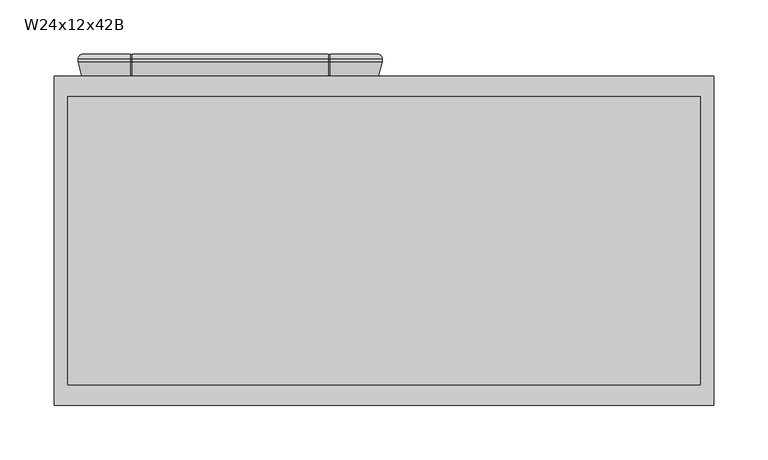
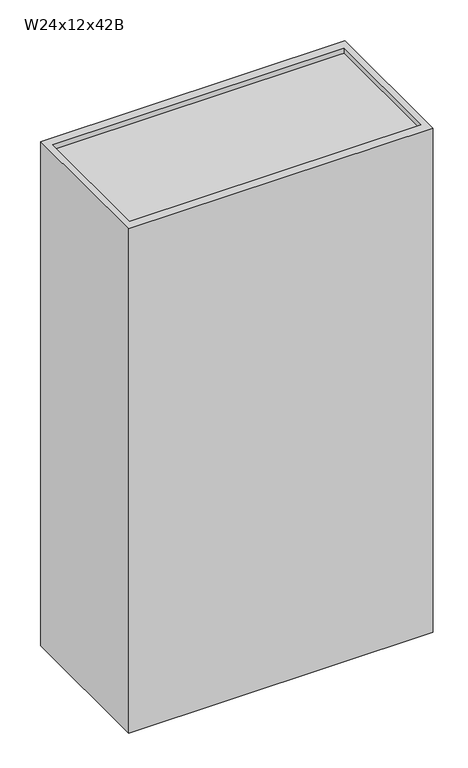
"""IFC4 building model written with IfcOpenShell, lengths in millimetres: furniture geometry, Cabinet-Wall-Merillat-Double_Door-Marlin : W24x12x42B."""

from ifc_helpers import new_model, si_unit, frame, origin, place, context, project, spatial, polyline, circle_curve, ellipse_curve, outline, extrude, faceted_brep, source, transform, mapped, element, save
from ifc_brep_helpers import plane_surface, cylinder_surface, advanced_brep


def w24x12x42b_d67e2903(model_context):
    return source(origin(), model_context, "Body", "SolidModel", [
        advanced_brep(
        [(-24.0971608, 382.5621, 2108.2), (-21.0006683, 387.0325, 2105.1035075), (-21.0006683, 387.0325, 1095.2964925), (-24.0971608, 382.5621, 1092.2), (-24.0971608, 379.7935, 1092.2), (-24.0971608, 379.7935, 2108.2), (-20.5919608, 366.7125, 1095.7052), (-20.5919608, 366.7125, 2104.6948), (24.104002, 366.7125, 2059.9988372), (24.104002, 366.7125, 1140.4011628), (24.4741337, 367.50625, 1140.7712945), (26.5552927, 371.96931, 1142.8524535), (26.5552927, 371.96931, 2057.5475465), (24.4741337, 367.50625, 2059.6287055), (25.1555233, 374.2094093, 1141.452684), (25.1555233, 374.2094093, 2058.947316), (10.8278392, 374.4595, 1127.125), (10.8278392, 374.4595, 2073.275), (10.8278392, 379.2855, 1127.125), (10.8278392, 379.2855, 2073.275), (25.1555233, 379.5355907, 1141.452684), (25.1555233, 379.5355907, 2058.947316), (26.5552927, 381.77569, 1142.8524535), (26.5552927, 381.77569, 2057.5475465), (24.4741337, 386.23875, 1140.7712945), (24.1068694, 387.0263508, 1140.4040302), (24.104002, 387.0325, 2059.9988372), (24.4741337, 386.23875, 2059.6287055), (24.1068694, 387.0325, 1095.2964925), (24.1068694, 382.5621, 1092.2), (253.7938467, 387.0325, 1095.2964925), (256.8903392, 382.5621, 1092.2), (208.7261206, 382.5621, 1092.2), (208.7261206, 387.0325, 1095.2964925), (25.6943694, 382.5621, 1092.2), (25.6943694, 387.0325, 1095.2964925), (207.1386206, 387.0325, 1095.2964925), (207.1386206, 382.5621, 1092.2), (24.1068694, 379.7935, 1092.2), (256.8903392, 379.7935, 1092.2), (208.7261206, 379.7935, 1092.2), (25.6943694, 379.7935, 1092.2), (207.1386206, 379.7935, 1092.2), (24.1068694, 366.7125, 1095.7052), (253.3851392, 366.7125, 1095.7052), (208.7261206, 366.7125, 1095.7052), (25.6943694, 366.7125, 1095.7052), (207.1386206, 366.7125, 1095.7052), (206.2378857, 371.96931, 1142.8524535), (25.6943694, 367.50625, 1140.7712945), (25.6943694, 366.7125, 1140.4011628), (207.1386206, 366.7125, 1140.4011628), (207.1386206, 367.50625, 1140.7712945), (208.3190448, 367.50625, 1140.7712945), (207.6376552, 374.2094093, 1141.452684), (221.9653392, 374.4595, 1127.125), (221.9653392, 379.2855, 1127.125), (207.6376552, 379.5355907, 1141.452684), (206.2378857, 381.77569, 1142.8524535), (208.3190448, 386.23875, 1140.7712945), (207.1386206, 386.23875, 1140.7712945), (207.1386206, 387.0325, 1140.4011628), (25.6943694, 387.0325, 1140.4011628), (25.6943694, 386.23875, 1140.7712945), (253.7938467, 387.0325, 2105.1035075), (256.8903392, 382.5621, 2108.2), (256.8903392, 379.7935, 2108.2), (253.3851392, 366.7125, 2104.6948), (208.6891765, 366.7125, 1140.4011628), (208.6891765, 366.7125, 2059.9988372), (208.3190448, 367.50625, 2059.6287055), (206.2378857, 371.96931, 2057.5475465), (207.6376552, 374.2094093, 2058.947316), (221.9653392, 374.4595, 2073.275), (221.9653392, 379.2855, 2073.275), (207.6376552, 379.5355907, 2058.947316), (206.2378857, 381.77569, 2057.5475465), (208.3190448, 386.23875, 2059.6287055), (208.6891765, 387.0325, 2059.9988372), (208.6891765, 387.0325, 1140.4011628), (208.7261206, 387.0325, 2105.1035075), (208.7261206, 382.5621, 2108.2), (24.1068694, 382.5621, 2108.2), (24.1068694, 387.0325, 2105.1035075), (207.1386206, 382.5621, 2108.2), (207.1386206, 387.0325, 2105.1035075), (25.6943694, 387.0325, 2105.1035075), (25.6943694, 382.5621, 2108.2), (208.7261206, 379.7935, 2108.2), (24.1068694, 379.7935, 2108.2), (207.1386206, 379.7935, 2108.2), (25.6943694, 379.7935, 2108.2), (208.7261206, 366.7125, 2104.6948), (24.1068694, 366.7125, 2104.6948), (207.1386206, 366.7125, 2104.6948), (25.6943694, 366.7125, 2104.6948), (207.1386206, 366.7125, 2059.9988372), (25.6943694, 366.7125, 2059.9988372), (207.1386206, 367.50625, 2059.6287055), (25.6943694, 367.50625, 2059.6287055), (25.6943694, 386.23875, 2059.6287055), (25.6943694, 387.0325, 2059.9988372), (207.1386206, 387.0325, 2059.9988372), (207.1386206, 386.23875, 2059.6287055), (207.1386206, 367.50625, 2104.0857412), (207.1386206, 379.8980037, 2107.40625), (207.1386206, 382.5621, 2107.40625), (207.1386206, 386.23875, 2104.9526052), (208.7261206, 386.23875, 2059.6287055), (208.7261206, 386.23875, 2104.9526052), (208.7261206, 382.5621, 2107.40625), (208.7261206, 379.8980037, 2107.40625), (208.7261206, 367.50625, 2104.0857412), (208.7261206, 367.50625, 2059.6287055), (24.1068694, 367.50625, 2059.6287055), (24.1068694, 367.50625, 2104.0857412), (24.1068694, 379.8980037, 2107.40625), (24.1068694, 382.5621, 2107.40625), (24.1068694, 386.23875, 2104.9526052), (24.1068694, 386.23875, 2059.6287055), (25.6943694, 386.23875, 2104.9526052), (25.6943694, 382.5621, 2107.40625), (25.6943694, 379.8980037, 2107.40625), (25.6943694, 367.50625, 2104.0857412), (24.1068694, 386.23875, 1140.7712945), (24.1068694, 386.23875, 1095.4473948), (24.1068694, 382.5621, 1092.99375), (24.1068694, 379.8980037, 1092.99375), (24.1068694, 367.50625, 1096.3142588), (24.1068694, 367.50625, 1140.7712945), (25.6943694, 367.50625, 1096.3142588), (25.6943694, 379.8980037, 1092.99375), (25.6943694, 382.5621, 1092.99375), (25.6943694, 386.23875, 1095.4473948), (207.1386206, 386.23875, 1095.4473948), (207.1386206, 382.5621, 1092.99375), (207.1386206, 379.8980037, 1092.99375), (207.1386206, 367.50625, 1096.3142588), (208.7261206, 386.23875, 1140.7712945), (208.7261206, 367.50625, 1140.7712945), (208.7261206, 367.50625, 1096.3142588), (208.7261206, 379.8980037, 1092.99375), (208.7261206, 382.5621, 1092.99375), (208.7261206, 386.23875, 1095.4473948)],
        [
            (0, 1, ellipse_curve(frame((-19.3219608, 382.5621, 2103.4248), z_axis=(-0.7071067811865475, 0.0, -0.7071067811865475), x_axis=(-0.7071067811865474, 0.0, 0.7071067811865476)), 6.7531526, 4.7752)),
            (1, 2),
            (2, 3, ellipse_curve(frame((-19.3219608, 382.5621, 1096.9752), z_axis=(-0.7071067811865475, 0.0, 0.7071067811865475), x_axis=(0.7071067811865474, 0.0, 0.7071067811865476)), 6.7531526, 4.7752)),
            (3, 0),
            (3, 4),
            (4, 5),
            (5, 0),
            (4, 6),
            (6, 7),
            (7, 5),
            (8, 9),
            (9, 10),
            (10, 11),
            (11, 12),
            (12, 13),
            (13, 8),
            (11, 14, ellipse_curve(frame((25.1280392, 372.6348492, 1141.4252), z_axis=(-0.7071067811865475, 0.0, 0.7071067811865475), x_axis=(0.7071067811865474, 0.0, 0.7071067811865476)), 2.2271035, 1.5748)),
            (14, 15),
            (15, 12, ellipse_curve(frame((25.1280392, 372.6348492, 2058.9748), z_axis=(-0.7071067811865475, 0.0, -0.7071067811865475), x_axis=(-0.7071067811865474, 0.0, 0.7071067811865476)), 2.2271035, 1.5748)),
            (14, 16),
            (16, 17),
            (17, 15),
            (16, 18),
            (18, 19),
            (19, 17),
            (18, 20),
            (20, 21),
            (21, 19),
            (20, 22, ellipse_curve(frame((25.1280392, 381.1101508, 1141.4252), z_axis=(-0.7071067811865475, 0.0, 0.7071067811865475), x_axis=(0.7071067811865474, 0.0, 0.7071067811865476)), 2.2271035, 1.5748)),
            (22, 23),
            (23, 21, ellipse_curve(frame((25.1280392, 381.1101508, 2058.9748), z_axis=(-0.7071067811865475, 0.0, -0.7071067811865475), x_axis=(-0.7071067811865474, 0.0, 0.7071067811865476)), 2.2271035, 1.5748)),
            (22, 24),
            (24, 25),
            (25, 26),
            (26, 27),
            (27, 23),
            (2, 28),
            (28, 29, circle_curve(frame((24.1068694, 382.5621, 1096.9752), z_axis=(-1.0, 0.0, 0.0), x_axis=(0.0, -1.0, 0.0)), 4.7752)),
            (29, 3),
            (30, 31, ellipse_curve(frame((252.1151392, 382.5621, 1096.9752), z_axis=(-0.7071067811865475, 0.0, -0.7071067811865475), x_axis=(-0.7071067811865476, 0.0, 0.7071067811865474)), 6.7531526, 4.7752)),
            (31, 32),
            (32, 33, circle_curve(frame((208.7261206, 382.5621, 1096.9752), z_axis=(1.0, 0.0, 0.0), x_axis=(0.0, -1.0, 0.0)), 4.7752)),
            (33, 30),
            (34, 35, circle_curve(frame((25.6943694, 382.5621, 1096.9752), z_axis=(1.0, 0.0, 0.0), x_axis=(0.0, -1.0, 0.0)), 4.7752)),
            (35, 36),
            (36, 37, circle_curve(frame((207.1386206, 382.5621, 1096.9752), z_axis=(-1.0, 0.0, 0.0), x_axis=(0.0, -1.0, 0.0)), 4.7752)),
            (37, 34),
            (29, 38),
            (38, 4),
            (31, 39),
            (39, 40),
            (40, 32),
            (41, 34),
            (37, 42),
            (42, 41),
            (38, 43),
            (43, 6),
            (39, 44),
            (44, 45),
            (45, 40),
            (46, 41),
            (42, 47),
            (47, 46),
            (48, 11),
            (10, 49),
            (49, 50),
            (50, 51),
            (51, 52),
            (52, 53),
            (53, 48),
            (48, 54, ellipse_curve(frame((207.6651392, 372.6348492, 1141.4252), z_axis=(-0.7071067811865475, 0.0, -0.7071067811865475), x_axis=(-0.7071067811865476, 0.0, 0.7071067811865474)), 2.2271035, 1.5748)),
            (54, 14),
            (54, 55),
            (55, 16),
            (55, 56),
            (56, 18),
            (56, 57),
            (57, 20),
            (57, 58, ellipse_curve(frame((207.6651392, 381.1101508, 1141.4252), z_axis=(-0.7071067811865475, 0.0, -0.7071067811865475), x_axis=(-0.7071067811865476, 0.0, 0.7071067811865474)), 2.2271035, 1.5748)),
            (58, 22),
            (58, 59),
            (59, 60),
            (60, 61),
            (61, 62),
            (62, 63),
            (63, 24),
            (30, 64),
            (64, 65, ellipse_curve(frame((252.1151392, 382.5621, 2103.4248), z_axis=(0.7071067811865475, 0.0, -0.7071067811865475), x_axis=(-0.7071067811865474, 0.0, -0.7071067811865476)), 6.7531526, 4.7752)),
            (65, 31),
            (65, 66),
            (66, 39),
            (66, 67),
            (67, 44),
            (68, 69),
            (69, 70),
            (70, 71),
            (71, 48),
            (53, 68),
            (71, 72, ellipse_curve(frame((207.6651392, 372.6348492, 2058.9748), z_axis=(0.7071067811865475, 0.0, -0.7071067811865475), x_axis=(-0.7071067811865474, 0.0, -0.7071067811865476)), 2.2271035, 1.5748)),
            (72, 54),
            (72, 73),
            (73, 55),
            (73, 74),
            (74, 56),
            (74, 75),
            (75, 57),
            (75, 76, ellipse_curve(frame((207.6651392, 381.1101508, 2058.9748), z_axis=(0.7071067811865475, 0.0, -0.7071067811865475), x_axis=(-0.7071067811865474, 0.0, -0.7071067811865476)), 2.2271035, 1.5748)),
            (76, 58),
            (76, 77),
            (77, 78),
            (78, 79),
            (79, 59),
            (64, 80),
            (80, 81, circle_curve(frame((208.7261206, 382.5621, 2103.4248), z_axis=(1.0, 0.0, 0.0), x_axis=(0.0, -1.0, 0.0)), 4.7752)),
            (81, 65),
            (0, 82),
            (82, 83, circle_curve(frame((24.1068694, 382.5621, 2103.4248), z_axis=(-1.0, 0.0, 0.0), x_axis=(0.0, -1.0, 0.0)), 4.7752)),
            (83, 1),
            (84, 85, circle_curve(frame((207.1386206, 382.5621, 2103.4248), z_axis=(-1.0, 0.0, 0.0), x_axis=(0.0, -1.0, 0.0)), 4.7752)),
            (85, 86),
            (86, 87, circle_curve(frame((25.6943694, 382.5621, 2103.4248), z_axis=(1.0, 0.0, 0.0), x_axis=(0.0, -1.0, 0.0)), 4.7752)),
            (87, 84),
            (81, 88),
            (88, 66),
            (5, 89),
            (89, 82),
            (90, 84),
            (87, 91),
            (91, 90),
            (88, 92),
            (92, 67),
            (7, 93),
            (93, 89),
            (94, 90),
            (91, 95),
            (95, 94),
            (43, 9),
            (8, 93),
            (92, 69),
            (68, 45),
            (96, 94),
            (95, 97),
            (97, 96),
            (50, 46),
            (47, 51),
            (12, 71),
            (70, 98),
            (98, 96),
            (97, 99),
            (99, 13),
            (15, 72),
            (17, 73),
            (19, 74),
            (21, 75),
            (23, 76),
            (27, 100),
            (100, 101),
            (101, 102),
            (102, 103),
            (103, 77),
            (83, 26),
            (25, 28),
            (33, 79),
            (78, 80),
            (85, 102),
            (101, 86),
            (35, 62),
            (61, 36),
            (98, 104),
            (104, 105),
            (105, 106),
            (106, 107, circle_curve(frame((207.1386206, 382.5621, 2103.4248), z_axis=(-1.0, 0.0, 0.0), x_axis=(0.0, 0.0, 1.0)), 3.98145)),
            (107, 103),
            (78, 108),
            (108, 109),
            (109, 110, circle_curve(frame((208.7261206, 382.5621, 2103.4248), z_axis=(1.0, 0.0, 0.0), x_axis=(0.0, 0.0, 1.0)), 3.98145)),
            (110, 111),
            (111, 112),
            (112, 113),
            (113, 69),
            (77, 108),
            (107, 109),
            (106, 110),
            (105, 111),
            (104, 112),
            (70, 113),
            (8, 114),
            (114, 115),
            (115, 116),
            (116, 117),
            (117, 118, circle_curve(frame((24.1068694, 382.5621, 2103.4248), z_axis=(-1.0, 0.0, 0.0), x_axis=(0.0, 0.0, 1.0)), 3.98145)),
            (118, 119),
            (119, 26),
            (100, 120),
            (120, 121, circle_curve(frame((25.6943694, 382.5621, 2103.4248), z_axis=(1.0, 0.0, 0.0), x_axis=(0.0, 0.0, 1.0)), 3.98145)),
            (121, 122),
            (122, 123),
            (123, 99),
            (119, 27),
            (118, 120),
            (117, 121),
            (116, 122),
            (115, 123),
            (114, 13),
            (25, 124),
            (124, 125),
            (125, 126, circle_curve(frame((24.1068694, 382.5621, 1096.9752), z_axis=(-1.0, 0.0, 0.0), x_axis=(0.0, 0.0, 1.0)), 3.98145)),
            (126, 127),
            (127, 128),
            (128, 129),
            (129, 9),
            (49, 130),
            (130, 131),
            (131, 132),
            (132, 133, circle_curve(frame((25.6943694, 382.5621, 1096.9752), z_axis=(1.0, 0.0, 0.0), x_axis=(0.0, 0.0, 1.0)), 3.98145)),
            (133, 63),
            (129, 10),
            (128, 130),
            (127, 131),
            (126, 132),
            (125, 133),
            (124, 24),
            (60, 134),
            (134, 135, circle_curve(frame((207.1386206, 382.5621, 1096.9752), z_axis=(-1.0, 0.0, 0.0), x_axis=(0.0, 0.0, 1.0)), 3.98145)),
            (135, 136),
            (136, 137),
            (137, 52),
            (138, 79),
            (68, 139),
            (139, 140),
            (140, 141),
            (141, 142),
            (142, 143, circle_curve(frame((208.7261206, 382.5621, 1096.9752), z_axis=(1.0, 0.0, 0.0), x_axis=(0.0, 0.0, 1.0)), 3.98145)),
            (143, 138),
            (138, 59),
            (53, 139),
            (137, 140),
            (136, 141),
            (135, 142),
            (134, 143),
        ],
        [
            cylinder_surface(frame((-19.3219608, 382.5621, 2108.2), z_axis=(0.0, 0.0, 1.0), x_axis=(0.0, -1.0, 0.0)), 4.7752),
            plane_surface(frame((-24.0971608, 382.5621, 2108.2), z_axis=(-1.0, 0.0, 0.0), x_axis=(0.0, 0.0, -1.0))),
            plane_surface(frame((-24.0971608, 379.7935, 2108.2), z_axis=(-0.9659229350723619, -0.25882983502910506, 0.0), x_axis=(0.0, 0.0, -1.0))),
            plane_surface(frame((24.104002, 366.7125, 2059.9988372), z_axis=(0.9063077870366099, -0.4226182617407856, 0.0), x_axis=(0.0, 0.0, -1.0))),
            cylinder_surface(frame((25.1280392, 372.6348492, 2108.2), z_axis=(0.0, 0.0, 1.0000000000000002), x_axis=(0.01745240643729364, 0.9998476951563912, 0.0)), 1.5748),
            plane_surface(frame((25.1555233, 374.2094093, 2058.947316), z_axis=(0.017452406437322144, 0.9998476951563906, 0.0), x_axis=(0.0, 0.0, -1.0))),
            plane_surface(frame((10.8278392, 374.4595, 2073.275), z_axis=(1.0, 0.0, 0.0), x_axis=(0.0, 0.0, -1.0))),
            plane_surface(frame((10.8278392, 379.2855, 2073.275), z_axis=(0.01745240643727848, -0.9998476951563914, 0.0), x_axis=(0.0, 0.0, -1.0))),
            cylinder_surface(frame((25.1280392, 381.1101508, 2108.2), z_axis=(0.0, 0.0, 1.0000000000000002), x_axis=(0.9063077870367326, 0.42261826174052236, 0.0)), 1.5748),
            plane_surface(frame((26.5552927, 381.77569, 2057.5475465), z_axis=(0.9063077870366333, 0.4226182617407352, 0.0), x_axis=(0.0, 0.0, -1.0))),
            cylinder_surface(frame((-24.0971608, 382.5621, 1096.9752), z_axis=(-1.0, 0.0, 0.0), x_axis=(0.0, -1.0, 0.0)), 4.7752),
            plane_surface(frame((-24.0971608, 382.5621, 1092.2), z_axis=(0.0, 0.0, -1.0), x_axis=(1.0, 0.0, 0.0))),
            plane_surface(frame((-24.0971608, 379.7935, 1092.2), z_axis=(0.0, -0.2588298350291095, -0.9659229350723607), x_axis=(1.0, 0.0, 0.0))),
            plane_surface(frame((24.104002, 366.7125, 1140.4011628), z_axis=(0.0, -0.42261826174078143, 0.9063077870366119), x_axis=(1.0, 0.0, 0.0))),
            cylinder_surface(frame((-24.0971608, 372.6348492, 1141.4252), z_axis=(-1.0000000000000002, 0.0, 0.0), x_axis=(0.0, 0.9998476951563913, 0.017452406437289025)), 1.5748),
            plane_surface(frame((25.1555233, 374.2094093, 1141.452684), z_axis=(0.0, 0.9998476951563907, 0.01745240643731753), x_axis=(1.0, 0.0, 0.0))),
            plane_surface(frame((10.8278392, 374.4595, 1127.125), z_axis=(0.0, 0.0, 1.0), x_axis=(1.0, 0.0, 0.0))),
            plane_surface(frame((10.8278392, 379.2855, 1127.125), z_axis=(0.0, -0.9998476951563913, 0.017452406437283095), x_axis=(1.0, 0.0, 0.0))),
            cylinder_surface(frame((-24.0971608, 381.1101508, 1141.4252), z_axis=(-1.0000000000000002, 0.0, 0.0), x_axis=(0.0, 0.4226182617405265, 0.9063077870367306)), 1.5748),
            plane_surface(frame((26.5552927, 381.77569, 1142.8524535), z_axis=(0.0, 0.4226182617407394, 0.9063077870366314), x_axis=(1.0, 0.0, 0.0))),
            cylinder_surface(frame((252.1151392, 382.5621, 1092.2), z_axis=(0.0, 0.0, -1.0), x_axis=(0.0, -1.0, 0.0)), 4.7752),
            plane_surface(frame((256.8903392, 382.5621, 1092.2), z_axis=(1.0, 0.0, 0.0), x_axis=(0.0, 0.0, 1.0))),
            plane_surface(frame((256.8903392, 379.7935, 1092.2), z_axis=(0.9659229350723619, -0.25882983502910506, 0.0), x_axis=(0.0, 0.0, 1.0))),
            plane_surface(frame((208.6891765, 366.7125, 1140.4011628), z_axis=(-0.9063077870366099, -0.4226182617407856, 0.0), x_axis=(0.0, 0.0, 1.0))),
            cylinder_surface(frame((207.6651392, 372.6348492, 1092.2), z_axis=(0.0, 0.0, -1.0000000000000002), x_axis=(-0.01745240643729364, 0.9998476951563912, 0.0)), 1.5748),
            plane_surface(frame((207.6376552, 374.2094093, 1141.452684), z_axis=(-0.017452406437322144, 0.9998476951563906, 0.0), x_axis=(0.0, 0.0, 1.0))),
            plane_surface(frame((221.9653392, 374.4595, 1127.125), z_axis=(-1.0, 0.0, 0.0), x_axis=(0.0, 0.0, 1.0))),
            plane_surface(frame((221.9653392, 379.2855, 1127.125), z_axis=(-0.01745240643727848, -0.9998476951563914, 0.0), x_axis=(0.0, 0.0, 1.0))),
            cylinder_surface(frame((207.6651392, 381.1101508, 1092.2), z_axis=(0.0, 0.0, -1.0000000000000002), x_axis=(-0.9063077870367326, 0.42261826174052236, 0.0)), 1.5748),
            plane_surface(frame((206.2378857, 381.77569, 1142.8524535), z_axis=(-0.9063077870366333, 0.4226182617407352, 0.0), x_axis=(0.0, 0.0, 1.0))),
            cylinder_surface(frame((256.8903392, 382.5621, 2103.4248), z_axis=(1.0, 0.0, 0.0), x_axis=(0.0, -1.0, 0.0)), 4.7752),
            plane_surface(frame((256.8903392, 382.5621, 2108.2), z_axis=(0.0, 0.0, 1.0), x_axis=(-1.0, 0.0, 0.0))),
            plane_surface(frame((256.8903392, 379.7935, 2108.2), z_axis=(0.0, -0.2588298350291006, 0.9659229350723632), x_axis=(-1.0, 0.0, 0.0))),
            plane_surface(frame((253.3851392, 366.7125, 2104.6948), z_axis=(0.0, -1.0, 0.0), x_axis=(-1.0, 0.0, 0.0))),
            plane_surface(frame((208.6891765, 366.7125, 2059.9988372), z_axis=(0.0, -0.42261826174078976, -0.9063077870366079), x_axis=(-1.0, 0.0, 0.0))),
            cylinder_surface(frame((256.8903392, 372.6348492, 2058.9748), z_axis=(1.0000000000000002, 0.0, 0.0), x_axis=(0.0, 0.999847695156391, -0.017452406437298253)), 1.5748),
            plane_surface(frame((207.6376552, 374.2094093, 2058.947316), z_axis=(0.0, 0.9998476951563905, -0.01745240643732676), x_axis=(-1.0, 0.0, 0.0))),
            plane_surface(frame((221.9653392, 374.4595, 2073.275), z_axis=(0.0, 0.0, -1.0), x_axis=(-1.0, 0.0, 0.0))),
            plane_surface(frame((221.9653392, 379.2855, 2073.275), z_axis=(0.0, -0.9998476951563915, -0.017452406437273867), x_axis=(-1.0, 0.0, 0.0))),
            cylinder_surface(frame((256.8903392, 381.1101508, 2058.9748), z_axis=(1.0000000000000002, 0.0, 0.0), x_axis=(0.0, 0.4226182617405182, -0.9063077870367346)), 1.5748),
            plane_surface(frame((206.2378857, 381.77569, 2057.5475465), z_axis=(0.0, 0.422618261740731, -0.9063077870366353), x_axis=(-1.0, 0.0, 0.0))),
            plane_surface(frame((208.6891765, 387.0325, 2059.9988372), z_axis=(0.0, 1.0, 0.0), x_axis=(-1.0, 0.0, 0.0))),
            plane_surface(frame((207.1386206, 387.0325, 2059.9988372), z_axis=(1.0, 0.0, 0.0), x_axis=(0.0, -0.9063077870366119, -0.4226182617407812))),
            plane_surface(frame((208.7261206, 387.0325, 2059.9988372), z_axis=(-1.0, 0.0, 0.0), x_axis=(0.0, 0.9063077870366119, 0.4226182617407812))),
            plane_surface(frame((207.1386206, 387.0325, 2059.9988372), z_axis=(0.0, -0.4226182617407812, 0.9063077870366119), x_axis=(1.0, 0.0, 0.0))),
            plane_surface(frame((207.1386206, 386.23875, 2059.6287055), z_axis=(0.0, 1.0, 0.0), x_axis=(1.0, 0.0, 0.0))),
            cylinder_surface(frame((208.7261206, 382.5621, 2103.4248), z_axis=(1.0, 0.0, 0.0), x_axis=(0.0, 0.0, 1.0)), 3.98145),
            plane_surface(frame((207.1386206, 382.5621, 2107.40625), z_axis=(0.0, 0.0, 1.0), x_axis=(1.0, 0.0, 0.0))),
            plane_surface(frame((207.1386206, 379.8980037, 2107.40625), z_axis=(0.0, -0.25882983502916007, 0.9659229350723473), x_axis=(1.0, 0.0, 0.0))),
            plane_surface(frame((207.1386206, 367.50625, 2104.0857412), z_axis=(0.0, -1.0, 0.0), x_axis=(1.0, 0.0, 0.0))),
            plane_surface(frame((207.1386206, 367.50625, 2059.6287055), z_axis=(0.0, 0.4226182617408151, 0.906307787036596), x_axis=(1.0, 0.0, 0.0))),
            plane_surface(frame((24.1068694, 387.0325, 2059.9988372), z_axis=(1.0, 0.0, 0.0), x_axis=(0.0, -0.9063077870366119, -0.4226182617407812))),
            plane_surface(frame((25.6943694, 387.0325, 2059.9988372), z_axis=(-1.0, 0.0, 0.0), x_axis=(0.0, 0.9063077870366119, 0.4226182617407812))),
            plane_surface(frame((24.1068694, 387.0325, 2059.9988372), z_axis=(0.0, -0.4226182617407812, 0.9063077870366119), x_axis=(1.0, 0.0, 0.0))),
            plane_surface(frame((24.1068694, 386.23875, 2059.6287055), z_axis=(0.0, 1.0, 0.0), x_axis=(1.0, 0.0, 0.0))),
            cylinder_surface(frame((25.6943694, 382.5621, 2103.4248), z_axis=(1.0, 0.0, 0.0), x_axis=(0.0, 0.0, 1.0)), 3.98145),
            plane_surface(frame((24.1068694, 382.5621, 2107.40625), z_axis=(0.0, 0.0, 1.0), x_axis=(1.0, 0.0, 0.0))),
            plane_surface(frame((24.1068694, 379.8980037, 2107.40625), z_axis=(0.0, -0.25882983502916257, 0.9659229350723466), x_axis=(1.0, 0.0, 0.0))),
            plane_surface(frame((24.1068694, 367.50625, 2104.0857412), z_axis=(0.0, -1.0, 0.0), x_axis=(1.0, 0.0, 0.0))),
            plane_surface(frame((24.1068694, 367.50625, 2059.6287055), z_axis=(0.0, 0.42261826174081607, 0.9063077870365956), x_axis=(1.0, 0.0, 0.0))),
            plane_surface(frame((24.1068694, 382.5621, 1101.7504), z_axis=(1.0, 0.0, 0.0), x_axis=(0.0, 1.0, 0.0))),
            plane_surface(frame((25.6943694, 382.5621, 1101.7504), z_axis=(-1.0, 0.0, 0.0), x_axis=(0.0, -1.0, 0.0))),
            plane_surface(frame((24.1068694, 366.7125, 1140.4011628), z_axis=(0.0, 0.4226182617407898, -0.906307787036608), x_axis=(1.0, 0.0, 0.0))),
            plane_surface(frame((24.1068694, 367.50625, 1140.7712945), z_axis=(0.0, -1.0, 0.0), x_axis=(1.0, 0.0, 0.0))),
            plane_surface(frame((24.1068694, 367.50625, 1096.3142588), z_axis=(0.0, -0.2588298350294553, -0.9659229350722681), x_axis=(1.0, 0.0, 0.0))),
            plane_surface(frame((24.1068694, 379.8980037, 1092.99375), z_axis=(0.0, 0.0, -1.0), x_axis=(1.0, 0.0, 0.0))),
            cylinder_surface(frame((25.6943694, 382.5621, 1096.9752), z_axis=(1.0, 0.0, 0.0), x_axis=(0.0, 0.0, 1.0)), 3.98145),
            plane_surface(frame((24.1068694, 386.23875, 1095.4473948), z_axis=(0.0, 1.0, 0.0), x_axis=(1.0, 0.0, 0.0))),
            plane_surface(frame((24.1068694, 386.23875, 1140.7712945), z_axis=(0.0, -0.42261826174079614, -0.9063077870366049), x_axis=(1.0, 0.0, 0.0))),
            plane_surface(frame((207.1386206, 386.23875, 1140.7712945), z_axis=(1.0000000000000002, 0.0, 0.0), x_axis=(0.0, 0.9063077870366271, -0.4226182617407486))),
            plane_surface(frame((208.7261206, 386.23875, 1140.7712945), z_axis=(-1.0000000000000002, 0.0, 0.0), x_axis=(0.0, -0.9063077870366271, 0.4226182617407486))),
            plane_surface(frame((207.1386206, 386.23875, 1140.7712945), z_axis=(0.0, -0.4226182617407486, -0.9063077870366271), x_axis=(1.0, 0.0, 0.0))),
            plane_surface(frame((207.1386206, 366.7125, 1140.4011628), z_axis=(0.0, 0.4226182617407898, -0.906307787036608), x_axis=(1.0, 0.0, 0.0))),
            plane_surface(frame((207.1386206, 367.50625, 1140.7712945), z_axis=(0.0, -1.0, 0.0), x_axis=(1.0, 0.0, 0.0))),
            plane_surface(frame((207.1386206, 367.50625, 1096.3142588), z_axis=(0.0, -0.25882983502945534, -0.9659229350722681), x_axis=(1.0, 0.0, 0.0))),
            plane_surface(frame((207.1386206, 379.8980037, 1092.99375), z_axis=(0.0, 0.0, -1.0), x_axis=(1.0, 0.0, 0.0))),
            cylinder_surface(frame((208.7261206, 382.5621, 1096.9752), z_axis=(1.0, 0.0, 0.0), x_axis=(0.0, 0.0, 1.0)), 3.98145),
            plane_surface(frame((207.1386206, 386.23875, 1095.4473948), z_axis=(0.0, 1.0, 0.0), x_axis=(1.0, 0.0, 0.0))),
        ],
        [
            (0, [[1, 2, 3, 4]]),
            (1, [[-4, 5, 6, 7]]),
            (2, [[-6, 8, 9, 10]]),
            (3, [[11, 12, 13, 14, 15, 16]]),
            (4, [[-14, 17, 18, 19]]),
            (5, [[-18, 20, 21, 22]]),
            (6, [[-21, 23, 24, 25]]),
            (7, [[-24, 26, 27, 28]]),
            (8, [[-27, 29, 30, 31]]),
            (9, [[-30, 32, 33, 34, 35, 36]]),
            (10, [[-3, 37, 38, 39]]),
            (10, [[40, 41, 42, 43]]),
            (10, [[44, 45, 46, 47]]),
            (11, [[-5, -39, 48, 49]]),
            (11, [[50, 51, 52, -41]]),
            (11, [[53, -47, 54, 55]]),
            (12, [[-8, -49, 56, 57]]),
            (12, [[58, 59, 60, -51]]),
            (12, [[61, -55, 62, 63]]),
            (13, [[64, -13, 65, 66, 67, 68, 69, 70]]),
            (14, [[-17, -64, 71, 72]]),
            (15, [[-20, -72, 73, 74]]),
            (16, [[-23, -74, 75, 76]]),
            (17, [[-26, -76, 77, 78]]),
            (18, [[-29, -78, 79, 80]]),
            (19, [[-80, 81, 82, 83, 84, 85, 86, -32]]),
            (20, [[-40, 87, 88, 89]]),
            (21, [[-50, -89, 90, 91]]),
            (22, [[-58, -91, 92, 93]]),
            (23, [[94, 95, 96, 97, -70, 98]]),
            (24, [[-71, -97, 99, 100]]),
            (25, [[-73, -100, 101, 102]]),
            (26, [[-75, -102, 103, 104]]),
            (27, [[-77, -104, 105, 106]]),
            (28, [[-79, -106, 107, 108]]),
            (29, [[-108, 109, 110, 111, 112, -81]]),
            (30, [[-88, 113, 114, 115]]),
            (30, [[-1, 116, 117, 118]]),
            (30, [[119, 120, 121, 122]]),
            (31, [[-90, -115, 123, 124]]),
            (31, [[-7, 125, 126, -116]]),
            (31, [[127, -122, 128, 129]]),
            (32, [[-92, -124, 130, 131]]),
            (32, [[-10, 132, 133, -125]]),
            (32, [[134, -129, 135, 136]]),
            (33, [[-9, -57, 137, -11, 138, -132]]),
            (33, [[-93, -131, 139, -94, 140, -59]]),
            (33, [[141, -136, 142, 143]]),
            (33, [[144, -63, 145, -67]]),
            (34, [[146, -96, 147, 148, -143, 149, 150, -15]]),
            (35, [[-19, 151, -99, -146]]),
            (36, [[-22, 152, -101, -151]]),
            (37, [[-25, 153, -103, -152]]),
            (38, [[-28, 154, -105, -153]]),
            (39, [[-31, 155, -107, -154]]),
            (40, [[-155, -36, 156, 157, 158, 159, 160, -109]]),
            (41, [[-2, -118, 161, -34, 162, -37]]),
            (41, [[-87, -43, 163, -111, 164, -113]]),
            (41, [[165, -158, 166, -120]]),
            (41, [[167, -84, 168, -45]]),
            (42, [[169, 170, 171, 172, 173, -159, -165, -119, -127, -134, -141, -148]]),
            (43, [[174, 175, 176, 177, 178, 179, 180, -139, -130, -123, -114, -164]]),
            (44, [[-174, -110, 181]]),
            (45, [[-173, 182, -175, -181, -160]]),
            (46, [[-172, 183, -176, -182]]),
            (47, [[-171, 184, -177, -183]]),
            (48, [[-170, 185, -178, -184]]),
            (49, [[-169, -147, 186, -179, -185]]),
            (50, [[-180, -186, -95]]),
            (51, [[187, 188, 189, 190, 191, 192, 193, -161, -117, -126, -133, -138]]),
            (52, [[194, 195, 196, 197, 198, -149, -142, -135, -128, -121, -166, -157]]),
            (53, [[-193, 199, -35]]),
            (54, [[-192, 200, -194, -156, -199]]),
            (55, [[-191, 201, -195, -200]]),
            (56, [[-190, 202, -196, -201]]),
            (57, [[-189, 203, -197, -202]]),
            (58, [[-188, 204, -150, -198, -203]]),
            (59, [[-187, -16, -204]]),
            (60, [[205, 206, 207, 208, 209, 210, 211, -137, -56, -48, -38, -162]]),
            (61, [[212, 213, 214, 215, 216, -85, -167, -44, -53, -61, -144, -66]]),
            (62, [[-211, 217, -12]]),
            (63, [[-210, 218, -212, -65, -217]]),
            (64, [[-209, 219, -213, -218]]),
            (65, [[-208, 220, -214, -219]]),
            (66, [[-207, 221, -215, -220]]),
            (67, [[-206, 222, -86, -216, -221]]),
            (68, [[-205, -33, -222]]),
            (69, [[223, 224, 225, 226, 227, -68, -145, -62, -54, -46, -168, -83]]),
            (70, [[228, -163, -42, -52, -60, -140, 229, 230, 231, 232, 233, 234]]),
            (71, [[-228, 235, -112]]),
            (72, [[-229, -98, 236]]),
            (73, [[-227, 237, -230, -236, -69]]),
            (74, [[-226, 238, -231, -237]]),
            (75, [[-225, 239, -232, -238]]),
            (76, [[-224, 240, -233, -239]]),
            (77, [[-223, -82, -235, -234, -240]]),
        ],
    ),
        extrude(outline(polyline([(221.9653392, 379.2855), (221.9653392, 374.4595), (10.8278392, 374.4595), (10.8278392, 379.2855), (221.9653392, 379.2855)])), frame((0.0, 0.0, 1127.125), z_axis=(0.0, 0.0, 1.0), x_axis=(1.0, 0.0, 0.0)), (0.0, 0.0, 1.0), 946.15),
        extrude(outline(polyline([(-8.5711577, 347.6625), (525.0128185, 347.6625), (525.0128185, 80.9625), (-8.5711577, 80.9625), (-8.5711577, 347.6625)])), frame((0.0, 0.0, 1876.425), z_axis=(0.0, 0.0, 1.0), x_axis=(1.0, 0.0, 0.0)), (0.0, 0.0, 1.0), 19.05),
        extrude(outline(polyline([(-8.5711577, 347.6625), (525.0128185, 347.6625), (525.0128185, 80.9625), (-8.5711577, 80.9625), (-8.5711577, 347.6625)])), frame((0.0, 0.0, 1304.925), z_axis=(0.0, 0.0, 1.0), x_axis=(1.0, 0.0, 0.0)), (0.0, 0.0, 1.0), 19.05),
        extrude(outline(polyline([(-8.5711577, 347.6625), (525.0128185, 347.6625), (525.0128185, 80.9625), (-8.5711577, 80.9625), (-8.5711577, 347.6625)])), frame((0.0, 0.0, 1590.675), z_axis=(0.0, 0.0, 1.0), x_axis=(1.0, 0.0, 0.0)), (0.0, 0.0, 1.0), 19.05),
        faceted_brep([(-46.3221608, 61.9125, 2133.6), (-46.3221608, 61.9125, 1066.8), (563.2778392, 61.9125, 1066.8), (563.2778392, 61.9125, 2133.6), (-46.3221608, 366.7125, 2133.6), (563.2778392, 366.7125, 2133.6), (563.2778392, 366.7125, 1066.8), (-46.3221608, 366.7125, 1066.8), (525.0128185, 366.7125, 2095.2735163), (301.9690685, 366.7125, 2095.2735163), (301.9690685, 366.7125, 1104.6672696), (525.0128185, 366.7125, 1104.6672696), (-8.5711577, 366.7125, 2095.2735163), (-8.5711577, 366.7125, 1104.6672696), (214.98661, 366.7125, 1104.6672696), (214.98661, 366.7125, 2095.2735163), (-33.6221608, 80.9625, 1066.8), (550.5778392, 80.9625, 1066.8), (550.5778392, 347.6625, 1066.8), (-33.6221608, 347.6625, 1066.8), (550.5778392, 347.6625, 2133.6), (550.5778392, 80.9625, 2133.6), (-33.6221608, 80.9625, 2133.6), (-33.6221608, 347.6625, 2133.6), (-8.5711577, 80.9625, 2095.2735163), (214.98661, 347.6625, 2095.2735163), (301.9690685, 347.6625, 2095.2735163), (525.0128185, 80.9625, 2095.2735163), (525.0128185, 80.9625, 1104.6672696), (301.9690685, 347.6625, 1104.6672696), (214.98661, 347.6625, 1104.6672696), (-8.5711577, 80.9625, 1104.6672696), (550.5778392, 80.9625, 2122.9851371), (550.5778392, 347.6625, 2122.9851371), (-33.6221608, 347.6625, 2122.9851371), (-33.6221608, 80.9625, 2122.9851371), (-33.6221608, 80.9625, 1076.6352657), (-33.6221608, 347.6625, 1076.6352657), (550.5778392, 347.6625, 1076.6352657), (550.5778392, 80.9625, 1076.6352657)], [[[0, 1, 2, 3]], [[4, 5, 6, 7], [8, 9, 10, 11], [12, 13, 14, 15]], [[1, 0, 4, 7]], [[2, 1, 7, 6], [16, 17, 18, 19]], [[3, 2, 6, 5]], [[0, 3, 5, 4], [20, 21, 22, 23]], [[24, 12, 15, 25, 26, 9, 8, 27]], [[8, 11, 28, 27]], [[28, 11, 10, 29, 30, 14, 13, 31]], [[13, 12, 24, 31]], [[32, 33, 34, 35]], [[33, 32, 21, 20]], [[34, 33, 20, 23]], [[35, 34, 23, 22]], [[32, 35, 22, 21]], [[36, 37, 38, 39]], [[36, 39, 17, 16]], [[39, 38, 18, 17]], [[38, 37, 19, 18]], [[37, 36, 16, 19]], [[24, 27, 28, 31]], [[26, 29, 10, 9]], [[15, 14, 30, 25]], [[29, 26, 25, 30]]]),
    ])


if __name__ == "__main__":
    model = new_model("IFC4")
    model_context = context("Model", 3, world=origin())
    ifc_project = project(units=[si_unit("LENGTHUNIT", "METRE", prefix="MILLI")], contexts=[model_context])
    site = spatial("IfcSite", under=ifc_project)
    building = spatial("IfcBuilding", under=site)
    placement = place(None, origin())
    w24x12x42b_shape = w24x12x42b_d67e2903(model_context)
    element("IfcFurniture", 1, ObjectType="Cabinet-Wall-Merillat-Double_Door-Marlin : W24x12x42B", at=placement, inside=building, context=model_context, shape_type="MappedRepresentation", body=[
        mapped(w24x12x42b_shape, transform((0.0, 0.0, 0.0), x_axis=(1.0, 0.0, 0.0), y_axis=(0.0, 1.0, 0.0), z_axis=(0.0, 0.0, 1.0))),
    ])
    save(model, "model.ifc")

# Revit data of these elements
# Type "Cabinet-Wall-Merillat-Double_Door-Marlin : W24x12x42B"
#   URL = "https://www.merillat.com/"
#   Product Page URL = "https://www.merillat.com/our-products/"
#   Product Line = "Express"
#   Product Group = "Wall Cabinet"
#   Product Documentation Link = "http://merillatbusiness.com/wp-content/uploads/2014/07/Merillat_Classic_Catalog.pdf"
#   Model = "W2442B"
#   Manufacturer = "Merillat"
#   Height Note = "Actual Height of 21 inches Cabinet is 20 1/2 inches"
#   Glass Door Note = "Glass Cabinet doors are only available in specific sizes. Please refer to the catalog for this information before requesting a glass size."
#   Finish = "Wood"
#   Description = "Wall 2442 Butt Door"
#   Construction Type = "Wall Cabinet"
#   Cabinet Construction Note = "Cabinets with B suffix have BUTT doors without a center frame stile:"
#   Assembly Code = "C1030410"
#   Spacing = 0' - 1"
#   Shelving Height = 0' - 9 3/4"
#   Door Spacing = 0' - 0 1/8"
#   Cabinet Door Width = 0' - 11 1/16"
#   Cabinet Door Height = 3' - 4"
#   Depth = 1' - 0"
#   Height = 3' - 6"
#   Top Of Cabinet = 7' - 0"
#   Width = 2' - 0"
#   COBie.Type = no
#   Top and Bottom Visibility = yes
#   Partial Overlay Butt = yes
#   Partial Overlay = no
#   Number of Shelves Greater than one = 3
#   Number of Shelves = 3
#   Middle Shelf = yes
#   Full Overlay Butt = no
#   Full Overlay = no
#   Elevation Swing Line = yes
#   Door Drawer Material = Wood - Merillat - Pecan(1)
#   Cabinet Material = Wood - Merillat - Pecan(1)
#   Cabinet Door Style = element 806847
# Element 1 (IfcFurniture, "Cabinet-Wall-Merillat-Double_Door-Marlin : W24x12x42B")
#   Materials on its faces: "Wood - Merillat - Pecan(1)"
# Materials
#   "Wood - Merillat - Pecan(1)": class "Wood", colour RGB 108 67 43, transparency 0, Cost = 0
